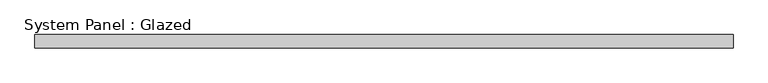
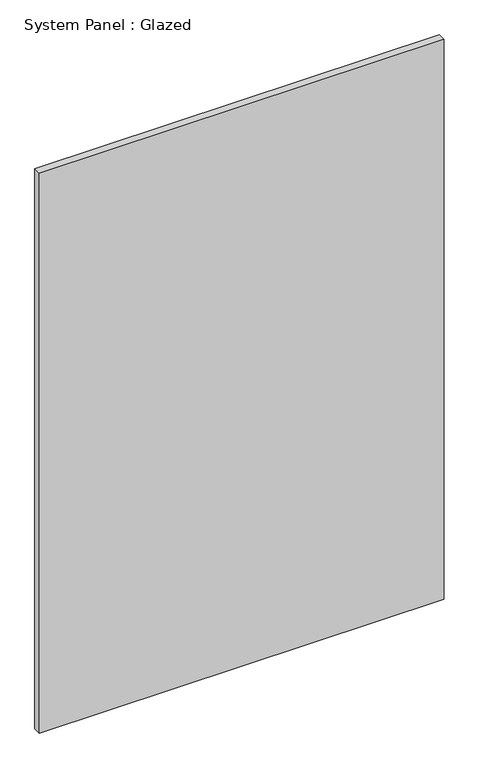
"""IFC4 building model written with IfcOpenShell, lengths in millimetres: plate geometry, System Panel : Glazed."""

from ifc_helpers import new_model, si_unit, origin, origin_with_axes, place, context, project, spatial, polyline, outline, extrude, source, transform, mapped, element, save


def system_panel_glazed_41482947(model_context):
    return source(origin(), model_context, "Body", "SweptSolid", [
        extrude(outline(polyline([(669.7103534, 19.05), (-669.7103534, 19.05), (-669.7103534, 44.45), (669.7103534, 44.45), (669.7103534, 19.05)])), origin_with_axes(), (0.0, 0.0, 1.0), 1957.9166667),
    ])


if __name__ == "__main__":
    model = new_model("IFC4")
    model_context = context("Model", 3, world=origin())
    ifc_project = project(units=[si_unit("LENGTHUNIT", "METRE", prefix="MILLI")], contexts=[model_context])
    site = spatial("IfcSite", under=ifc_project)
    building = spatial("IfcBuilding", under=site)
    placement = place(None, origin())
    system_panel_glazed_shape = system_panel_glazed_41482947(model_context)
    element("IfcPlate", 1, ObjectType="System Panel : Glazed", at=placement, inside=building, context=model_context, shape_type="MappedRepresentation", body=[
        mapped(system_panel_glazed_shape, transform((0.0, 0.0, 0.0), x_axis=(1.0, 0.0, 0.0), y_axis=(0.0, 1.0, 0.0), z_axis=(0.0, 0.0, 1.0))),
    ])
    save(model, "model.ifc")

# Revit data of these elements
# Type "System Panel : Glazed"
#   Construction Type Id = "GSP4R"
#   Analytic Construction = "1/8 in Pilkington single glazing"
#   Visual Light Transmittance = 0.9
#   Solar Heat Gain Coefficient = 0.86
#   Heat Transfer Coefficient (U) = 1.18115 BTU/(h·ft²·°F)
#   Define Thermal Properties by = 1
# Element 1 (IfcPlate, "System Panel : Glazed")
#   Materials on its faces: "Glass"
# Materials
#   "Glass": class "Glass", colour RGB 0 128 192, transparency 0.75, Description = "Soda Lime Glass", Cost = 0
